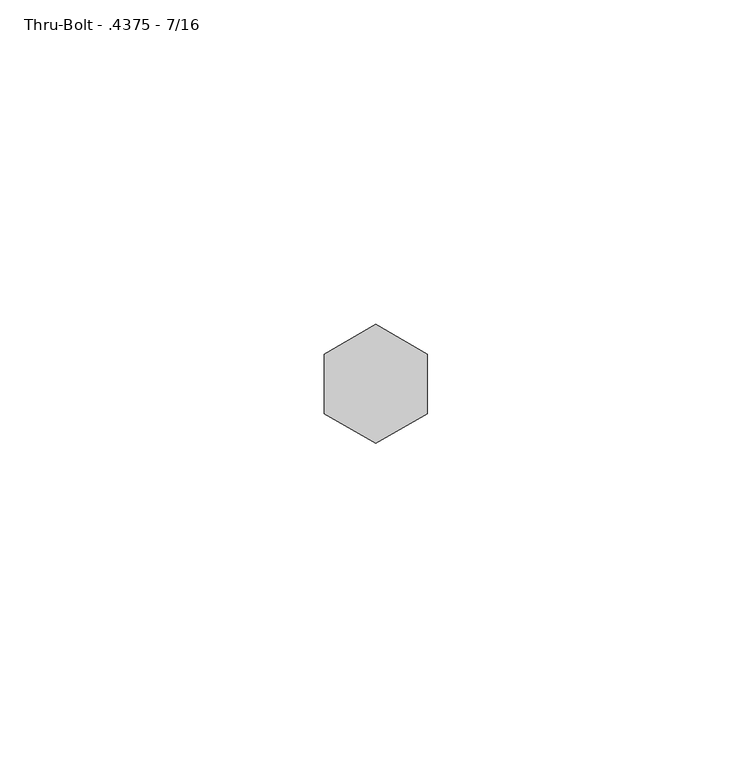
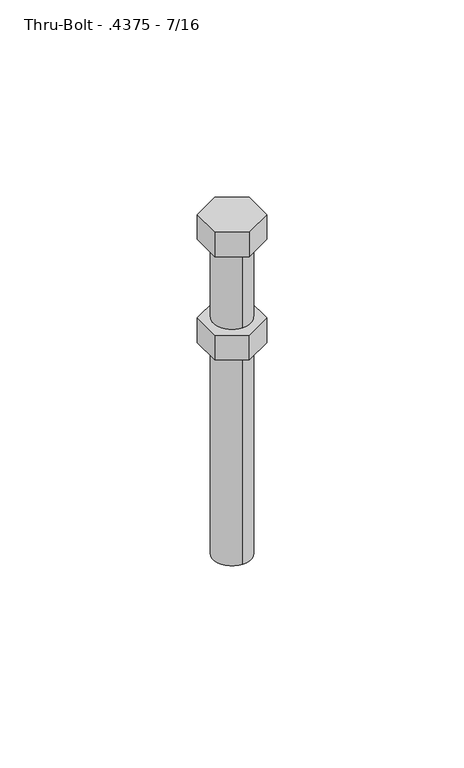
"""IFC4 building model written with IfcOpenShell, lengths in millimetres: fastener geometry, 060523 - W_P_C - Fastenings - Generic : Thru-Bolt - .4375 - 7/16."""

from ifc_helpers import new_model, si_unit, point, frame, origin, origin_with_axes, origin_2d, place, context, project, spatial, polyline, circle_curve, trimmed, segment, composite_curve, outline, extrude, source, transform, mapped, element, save


def thru_bolt_4375_7_16_993d5b58(model_context):
    return source(origin(), model_context, "Body", "SweptSolid", [
        extrude(outline(polyline([(-7.9375, -4.5827178), (-7.9375, 4.5827178), (0.0, 9.1654355), (7.9375, 4.5827178), (7.9375, -4.5827178), (0.0, -9.1654355), (-7.9375, -4.5827178)])), frame((0.0, 0.0, -33.4367188), z_axis=(0.0, 0.0, 1.0), x_axis=(1.0, 0.0, 0.0)), (0.0, 0.0, 1.0), 8.0367187),
        extrude(outline(polyline([(-7.9375, 4.5827178), (0.0, 9.1654355), (7.9375, 4.5827178), (7.9375, -4.5827178), (0.0, -9.1654355), (-7.9375, -4.5827178), (-7.9375, 4.5827178)])), origin_with_axes(), (0.0, 0.0, 1.0), 8.0367187),
        extrude(outline(composite_curve([segment(trimmed(circle_curve(origin_2d(), 5.7546875), [point((0.0, -5.7546875))], [point((0.0, 5.7546875))], False, "CARTESIAN"), True, "CONTINUOUS"), segment(trimmed(circle_curve(origin_2d(), 5.7546875), [point((0.0, 5.7546875))], [point((0.0, -5.7546875))], False, "CARTESIAN"), True, "CONTINUOUS")], self_intersect=False)), frame((0.0, 0.0, -101.6), z_axis=(0.0, 0.0, 1.0), x_axis=(1.0, 0.0, 0.0)), (0.0, 0.0, 1.0), 101.6),
    ])


if __name__ == "__main__":
    model = new_model("IFC4")
    model_context = context("Model", 3, world=origin())
    ifc_project = project(units=[si_unit("LENGTHUNIT", "METRE", prefix="MILLI")], contexts=[model_context])
    site = spatial("IfcSite", under=ifc_project)
    building = spatial("IfcBuilding", under=site)
    placement = place(None, origin())
    thru_bolt_4375_7_16_shape = thru_bolt_4375_7_16_993d5b58(model_context)
    element("IfcFastener", 1, ObjectType="060523 - W_P_C - Fastenings - Generic : Thru-Bolt - .4375 - 7/16", at=placement, inside=building, context=model_context, shape_type="MappedRepresentation", body=[
        mapped(thru_bolt_4375_7_16_shape, transform((0.0, 0.0, 0.0), x_axis=(1.0, 0.0, 0.0), y_axis=(0.0, 1.0, 0.0), z_axis=(0.0, 0.0, 1.0))),
    ])
    save(model, "model.ifc")

# Revit data of these elements
# Type "060523 - W_P_C - Fastenings - Generic : Thru-Bolt - .4375 - 7/16"
#   Washer_Thickness = 0' - 0 27/256"
#   Washer Radius = 0' - 0 139/256"
#   Washer Offset - Head = 0' - 0"
#   Washer Offset = 0' - 0"
#   Thickness_of_Substrate [instance default] = 0' - 1"
#   Side = 0' - 0.36133"
#   Radius = 0' - 0 29/128"
#   Length [instance default] = 0' - 4"
#   Head Size = 0' - 0 5/8"
#   Head Radius = 0' - 0 5/16"
#   Head Height = 0' - 0 81/256"
#   Double Diameter = 0' - 0 29/32"
#   Diameter = 0' - 0 29/64"
#   Default Elevation = 4' - 0"
#   Washer_Nut_Visibility = no
#   Washer_Head_Visibility = no
#   Round_Head_Visibility = no
#   Point Visibility = no
#   Nut_Visibility = yes
#   Hex_Head_Visiblilty = yes
#   Washer Material = none
#   Bolt Material (Size) = AT SILL - FASTENER AT 24" O.C.
# Element 1 (IfcFastener, "060523 - W_P_C - Fastenings - Generic : Thru-Bolt - .4375 - 7/16")
#   Materials on its faces: "AT SILL - FASTENER AT 24\" O.C."
# Materials
#   "AT SILL - FASTENER AT 24\" O.C.": class "Generic", colour RGB 120 120 120, transparency 0, Cost = 0
